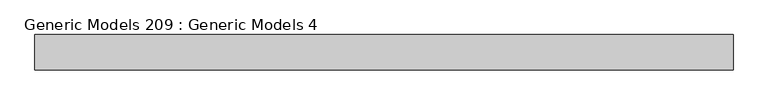
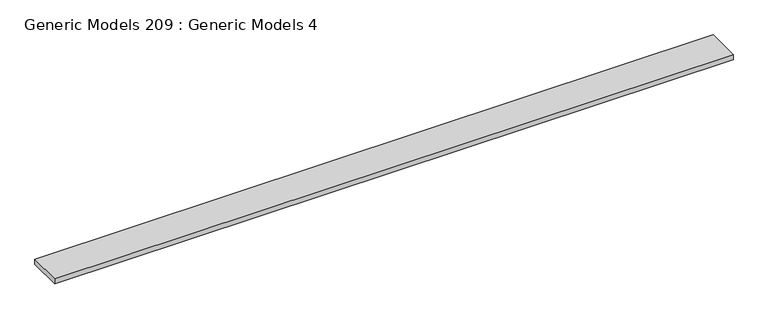
"""IFC4 building model written with IfcOpenShell, lengths in millimetres: proxy geometry, Generic Models 209 : Generic Models 4."""

from ifc_helpers import new_model, si_unit, frame, origin, place, context, project, spatial, polyline, outline, extrude, source, transform, mapped, element, save


def generic_models_209_generic_models_4_567cd659(model_context):
    return source(origin(), model_context, "Body", "SweptSolid", [
        extrude(outline(polyline([(-19489.9914237, 6242.3269221), (-19489.9914237, 6877.3269221), (-6942.3914237, 6877.3269221), (-6942.3914237, 6242.3269221), (-19489.9914237, 6242.3269221)])), frame((0.0, 0.0, 122856.628424), z_axis=(0.0, 0.0, 1.0), x_axis=(1.0, 0.0, 0.0)), (0.0, 0.0, 1.0), 101.6),
    ])


if __name__ == "__main__":
    model = new_model("IFC4")
    model_context = context("Model", 3, world=origin())
    ifc_project = project(units=[si_unit("LENGTHUNIT", "METRE", prefix="MILLI")], contexts=[model_context])
    site = spatial("IfcSite", under=ifc_project)
    building = spatial("IfcBuilding", under=site)
    placement = place(None, origin())
    generic_models_209_generic_models_4_shape = generic_models_209_generic_models_4_567cd659(model_context)
    element("IfcBuildingElementProxy", 1, Name="Generic Models 209 : Generic Models 4", ObjectType="Generic Models 209 : Generic Models 4", at=placement, inside=building, context=model_context, shape_type="MappedRepresentation", body=[
        mapped(generic_models_209_generic_models_4_shape, transform((0.0, 0.0, 0.0), x_axis=(1.0, 0.0, 0.0), y_axis=(0.0, 1.0, 0.0), z_axis=(0.0, 0.0, 1.0))),
    ])
    save(model, "model.ifc")

# Revit data of these elements
# Element 1 (IfcBuildingElementProxy, "Generic Models 209 : Generic Models 4")
#   Materials on its faces: "_4\" MIN. CRUSHED GRAVEL (NO FINES)"
# Materials
#   "_4\" MIN. CRUSHED GRAVEL (NO FINES)": class "Generic", colour RGB 122 131 148, transparency 0, Cost = 0
